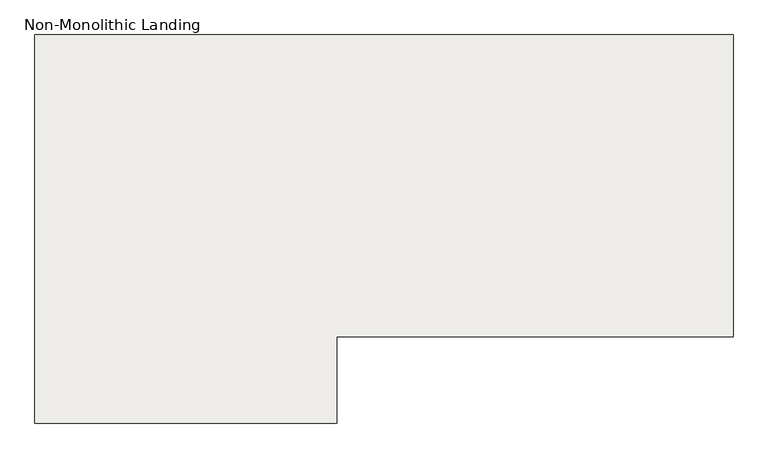
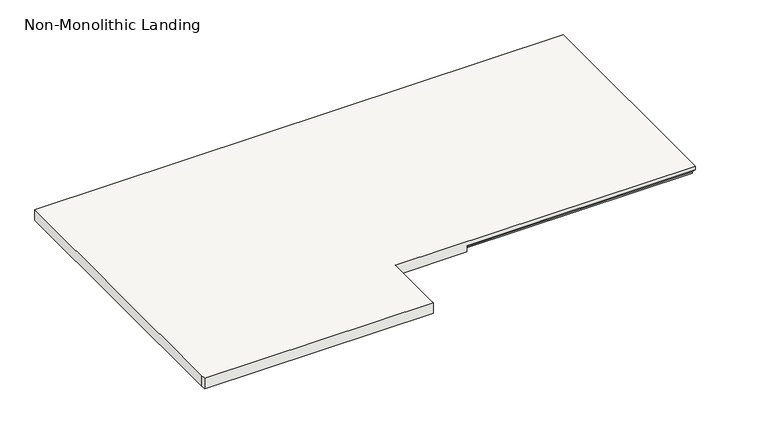
"""IFC4 building model written with IfcOpenShell, lengths in millimetres: slab geometry, Non-Monolithic Landing."""

from ifc_helpers import new_model, si_unit, origin, place, context, project, spatial, faceted_brep, source, transform, mapped, element, save


def non_monolithic_landing_f537d3a4(model_context):
    return source(origin(), model_context, "Body", "Brep", [
        faceted_brep([(-7676.1954607, 1223.3695005, 32555.8978261), (-7676.1954607, 1197.9695005, 32581.2978261), (-8742.9954607, 1197.9695005, 32581.2978261), (-8742.9954607, 1223.3695005, 32555.8978261), (-7676.1954607, 2264.7695005, 32600.3478261), (-10143.1704607, 2264.7695005, 32600.3478261), (-10143.1704607, 918.5695005, 32600.3478261), (-10143.1704607, 893.1695005, 32600.3478261), (-9076.3704607, 893.1695005, 32600.3478261), (-9076.3704607, 918.5695005, 32600.3478261), (-9076.3704607, 1197.9695005, 32600.3478261), (-7676.1954607, 1197.9695005, 32600.3478261), (-8742.9954607, 1223.3695005, 32549.5478261), (-8742.9954607, 1197.9695005, 32549.5478261), (-9076.3704607, 1197.9695005, 32549.5478261), (-9076.3704607, 918.5695005, 32549.5478261), (-9076.3704607, 893.1695005, 32549.5478261), (-10143.1704607, 893.1695005, 32549.5478261), (-10143.1704607, 918.5695005, 32549.5478261), (-10143.1704607, 2264.7695005, 32549.5478261), (-7676.1954607, 2264.7695005, 32549.5478261), (-7676.1954607, 1223.3695005, 32549.5478261)], [[[0, 1, 2, 3]], [[4, 5, 6, 7, 8, 9, 10, 11]], [[12, 13, 14, 15, 16, 17, 18, 19, 20, 21]], [[13, 12, 3, 2]], [[12, 21, 0, 3]], [[4, 11, 1, 0, 21, 20]], [[5, 4, 20, 19]], [[6, 5, 19, 18]], [[7, 6, 18, 17]], [[8, 7, 17, 16]], [[9, 8, 16, 15]], [[10, 9, 15, 14]], [[11, 10, 14, 13, 2, 1]]]),
    ])


if __name__ == "__main__":
    model = new_model("IFC4")
    model_context = context("Model", 3, world=origin())
    ifc_project = project(units=[si_unit("LENGTHUNIT", "METRE", prefix="MILLI")], contexts=[model_context])
    site = spatial("IfcSite", under=ifc_project)
    building = spatial("IfcBuilding", under=site)
    placement = place(None, origin())
    non_monolithic_landing_shape = non_monolithic_landing_f537d3a4(model_context)
    element("IfcSlab", 1, ObjectType="Non-Monolithic Landing", at=placement, inside=building, context=model_context, shape_type="MappedRepresentation", body=[
        mapped(non_monolithic_landing_shape, transform((0.0, 0.0, 0.0), x_axis=(1.0, 0.0, 0.0), y_axis=(0.0, 1.0, 0.0), z_axis=(0.0, 0.0, 1.0))),
    ])
    save(model, "model.ifc")
